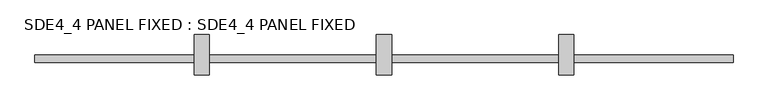
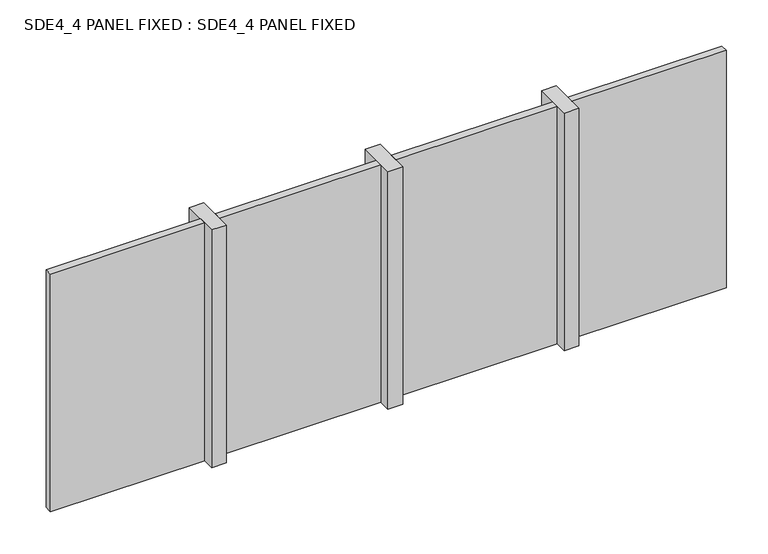
"""IFC4 building model written with IfcOpenShell, lengths in millimetres: plate geometry, SDE4_4 PANEL FIXED : SDE4_4 PANEL FIXED."""

from ifc_helpers import new_model, si_unit, origin, origin_with_axes, place, context, project, spatial, polyline, outline, extrude, source, transform, mapped, element, save


def sde4_4_panel_fixed_sde4_4_panel_fixed_4e835431(model_context):
    return source(origin(), model_context, "Body", "SweptSolid", [
        extrude(outline(polyline([(-1150.0, -132.5), (-1250.0, -132.5), (-1250.0, 132.5), (-1150.0, 132.5), (-1150.0, -132.5)])), origin_with_axes(), (0.0, 0.0, 1.0), 1710.0),
        extrude(outline(polyline([(50.0, -132.5), (-50.0, -132.5), (-50.0, 132.5), (50.0, 132.5), (50.0, -132.5)])), origin_with_axes(), (0.0, 0.0, 1.0), 1710.0),
        extrude(outline(polyline([(1250.0, -132.5), (1150.0, -132.5), (1150.0, 132.5), (1250.0, 132.5), (1250.0, -132.5)])), origin_with_axes(), (0.0, 0.0, 1.0), 1710.0),
        extrude(outline(polyline([(2299.0, -50.0), (1250.0, -50.0), (1250.0, 0.0), (2299.0, 0.0), (2299.0, -50.0)])), origin_with_axes(), (0.0, 0.0, 1.0), 1710.0),
        extrude(outline(polyline([(1150.0, -50.0), (50.0, -50.0), (50.0, 0.0), (1150.0, 0.0), (1150.0, -50.0)])), origin_with_axes(), (0.0, 0.0, 1.0), 1710.0),
        extrude(outline(polyline([(-50.0, -50.0), (-1150.0, -50.0), (-1150.0, 0.0), (-50.0, 0.0), (-50.0, -50.0)])), origin_with_axes(), (0.0, 0.0, 1.0), 1710.0),
        extrude(outline(polyline([(-1250.0, -50.0), (-2300.0, -50.0), (-2300.0, 0.0), (-1250.0, 0.0), (-1250.0, -50.0)])), origin_with_axes(), (0.0, 0.0, 1.0), 1710.0),
    ])


if __name__ == "__main__":
    model = new_model("IFC4")
    model_context = context("Model", 3, world=origin())
    ifc_project = project(units=[si_unit("LENGTHUNIT", "METRE", prefix="MILLI")], contexts=[model_context])
    site = spatial("IfcSite", under=ifc_project)
    building = spatial("IfcBuilding", under=site)
    placement = place(None, origin())
    sde4_4_panel_fixed_sde4_4_panel_fixed_shape = sde4_4_panel_fixed_sde4_4_panel_fixed_4e835431(model_context)
    element("IfcPlate", 1, ObjectType="SDE4_4 PANEL FIXED : SDE4_4 PANEL FIXED", at=placement, inside=building, context=model_context, shape_type="MappedRepresentation", body=[
        mapped(sde4_4_panel_fixed_sde4_4_panel_fixed_shape, transform((0.0, 0.0, 0.0), x_axis=(1.0, 0.0, 0.0), y_axis=(0.0, 1.0, 0.0), z_axis=(0.0, 0.0, 1.0))),
    ])
    save(model, "model.ifc")

# Revit data of these elements
# Type "SDE4_4 PANEL FIXED : SDE4_4 PANEL FIXED"
#   Type Mark = "CW-GLASS"
#   Analytic Construction = "<None>"
#   Glass = Glass
#   Frame = Aluminium
# Element 1 (IfcPlate, "SDE4_4 PANEL FIXED : SDE4_4 PANEL FIXED")
#   Materials on its faces: "Glass", "Aluminium"
# Materials
#   "Glass": class "Glass", colour RGB 0 128 192, transparency 0.9, Keynote = "L40", Cost = 0
#   "Aluminium": class "Unassigned", colour RGB 247 247 247, transparency 0, Cost = 0
